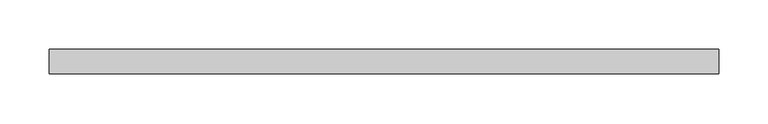
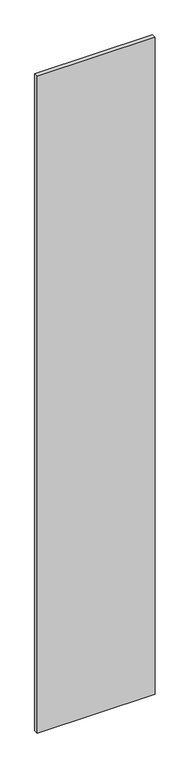
"""IFC4 building model written with IfcOpenShell, lengths in millimetres: plate geometry, 系统嵌板 : 玻璃."""

import ifcopenshell
import ifcopenshell.guid

model = None  # the IFC model being written
_history = None  # IfcOwnerHistory: only IFC2X3 demands one
_inside = {}  # id of a spatial element -> (the spatial element, [elements in it])
_under = {}  # id of a project, library or spatial element -> (it, [spatial elements below it])
_declared = {}  # id of a project -> (the project, [libraries it declares])
_typed = {}  # id of a type object -> (the type object, [elements of that type])
_made_of = {}  # id of a material, layer set ... -> (it, [elements and type objects made of it])


def new_model(schema):
    """Start an empty IFC model of exactly this schema.

    Asked for "IFC4X3", IfcOpenShell would pick the latest addendum, in which some entities
    have other attributes; the version numbers below select the first issue.
    IFC2X3 requires an IfcOwnerHistory on every rooted entity: one is made here for all.
    """
    global model, _history
    if schema == "IFC4X3":
        model = ifcopenshell.file(schema_version=(4, 3, 0, 0))
    else:
        model = ifcopenshell.file(schema=schema)
    _inside.clear()
    _under.clear()
    _declared.clear()
    _typed.clear()
    _made_of.clear()
    _history = None
    if model.schema == "IFC2X3":
        org = make("IfcOrganization", Name="unknown")
        user = make(
            "IfcPersonAndOrganization",
            ThePerson=make("IfcPerson", FamilyName="unknown"),
            TheOrganization=org,
        )
        app = make(
            "IfcApplication",
            ApplicationDeveloper=org,
            Version="unknown",
            ApplicationFullName="unknown",
            ApplicationIdentifier="unknown",
        )
        _history = make(
            "IfcOwnerHistory",
            OwningUser=user,
            OwningApplication=app,
            ChangeAction="ADDED",
            CreationDate=0,
        )
    return model


def make(cls, **values):
    """One entity of the class cls with the attributes given. An attribute that is None is left unset."""
    return model.create_entity(
        cls, **{name: value for name, value in values.items() if value is not None}
    )


def rooted(cls, **values):
    """An entity with a GlobalId (a new one), such as an element, a storey or a relation."""
    return make(cls, GlobalId=ifcopenshell.guid.new(), OwnerHistory=_history, **values)


def si_unit(unit_type, name, prefix=None):
    """IfcSIUnit, for example si_unit("LENGTHUNIT", "METRE", prefix="MILLI")."""
    return make("IfcSIUnit", UnitType=unit_type, Prefix=prefix, Name=name)


def assignment(units):
    """IfcUnitAssignment: the units of a project."""
    return None if units is None else make("IfcUnitAssignment", Units=units)


def point(xyz):
    """IfcCartesianPoint."""
    return None if xyz is None else make("IfcCartesianPoint", Coordinates=xyz)


def direction(xyz):
    """IfcDirection."""
    return None if xyz is None else make("IfcDirection", DirectionRatios=xyz)


def frame(location, z_axis=None, x_axis=None):
    """IfcAxis2Placement3D, a coordinate frame: its origin and axes. An axis left out is left unset."""
    return make(
        "IfcAxis2Placement3D",
        Location=point(location),
        Axis=direction(z_axis),
        RefDirection=direction(x_axis),
    )


def origin():
    """The frame at (0, 0, 0) with its axes left unset."""
    return frame((0.0, 0.0, 0.0))


def origin_with_axes():
    """The frame at (0, 0, 0) with the z axis (0, 0, 1) and the x axis (1, 0, 0) written out."""
    return frame((0.0, 0.0, 0.0), z_axis=(0.0, 0.0, 1.0), x_axis=(1.0, 0.0, 0.0))


def place(relative_to, where):
    """IfcLocalPlacement: puts the frame where relative to a parent placement (None: the world)."""
    return make(
        "IfcLocalPlacement", PlacementRelTo=relative_to, RelativePlacement=where
    )


def context(
    kind, dimensions, precision=None, world=None, true_north=None, identifier=None
):
    """IfcGeometricRepresentationContext, for example the 3D "Model" context."""
    return make(
        "IfcGeometricRepresentationContext",
        ContextIdentifier=identifier,
        ContextType=kind,
        CoordinateSpaceDimension=dimensions,
        Precision=precision,
        WorldCoordinateSystem=world,
        TrueNorth=true_north,
    )


def project(units=None, contexts=None):
    """IfcProject with its units and contexts."""
    return rooted(
        "IfcProject",
        Name="project",
        RepresentationContexts=contexts,
        UnitsInContext=assignment(units),
    )


def spatial(cls, under=None, at=None, **own):
    """A site, building, storey or space (cls), placed at a placement, below another one or the project."""
    s = rooted(cls, ObjectPlacement=at, **own)
    if under is not None:
        _under.setdefault(under.id(), (under, []))[1].append(s)
    return s


def polyline(points):
    """IfcPolyline through the points."""
    return make("IfcPolyline", Points=[point(p) for p in points])


def outline(outer, holes=None, kind="AREA"):
    """IfcArbitraryClosedProfileDef: a profile drawn as a closed curve; with holes, ...WithVoids."""
    if holes is None:
        return make("IfcArbitraryClosedProfileDef", ProfileType=kind, OuterCurve=outer)
    return make(
        "IfcArbitraryProfileDefWithVoids",
        ProfileType=kind,
        OuterCurve=outer,
        InnerCurves=holes,
    )


def extrude(swept, where, along, depth):
    """IfcExtrudedAreaSolid: the profile swept, set in the frame where, extruded along a direction by depth."""
    return make(
        "IfcExtrudedAreaSolid",
        SweptArea=swept,
        Position=where,
        ExtrudedDirection=direction(along),
        Depth=depth,
    )


def shape(context_of_items, identifier, shape_type, items):
    """IfcShapeRepresentation: the items that make up one representation, for example the "Body"."""
    return make(
        "IfcShapeRepresentation",
        ContextOfItems=context_of_items,
        RepresentationIdentifier=identifier,
        RepresentationType=shape_type,
        Items=items,
    )


def source(mapping_origin, context_of_items, identifier, shape_type, items):
    """IfcRepresentationMap: a shape defined once, which mapped items show again and again."""
    return make(
        "IfcRepresentationMap",
        MappingOrigin=mapping_origin,
        MappedRepresentation=shape(context_of_items, identifier, shape_type, items),
    )


def transform(
    local_origin,
    x_axis=None,
    y_axis=None,
    z_axis=None,
    scale=None,
    scale2=None,
    scale3=None,
    uniform=True,
):
    """IfcCartesianTransformationOperator3D, or its non-uniform kind. x_axis, y_axis, z_axis: its Axis1, 2, 3."""
    if uniform:
        return make(
            "IfcCartesianTransformationOperator3D",
            Axis1=direction(x_axis),
            Axis2=direction(y_axis),
            LocalOrigin=point(local_origin),
            Scale=scale,
            Axis3=direction(z_axis),
        )
    return make(
        "IfcCartesianTransformationOperator3DnonUniform",
        Axis1=direction(x_axis),
        Axis2=direction(y_axis),
        LocalOrigin=point(local_origin),
        Scale=scale,
        Axis3=direction(z_axis),
        Scale2=scale2,
        Scale3=scale3,
    )


def mapped(mapping_source, mapping_target):
    """IfcMappedItem: shows the shape of a source again, moved by a transform."""
    return make(
        "IfcMappedItem", MappingSource=mapping_source, MappingTarget=mapping_target
    )


def made_of(thing, what):
    """Note that an element or type object is made of a material, layer set ...; save() writes the relation."""
    if what is not None:
        _made_of.setdefault(what.id(), (what, []))[1].append(thing)
    return thing


def element(
    cls,
    number,
    at=None,
    inside=None,
    cuts=None,
    type_object=None,
    material=None,
    context=None,
    identifier="Body",
    shape_type=None,
    held_by="IfcProductDefinitionShape",
    body=None,
    shapes=None,
    **own,
):
    """One element of the class cls, such as IfcWall. Its Tag is "e" and its number.

    at: its placement. inside: the storey or other place that contains it. cuts: it is an
    opening in that element (IfcRelVoidsElement). A single representation is given by context,
    identifier, shape_type and body (its items); several are given by shapes. held_by: the class
    of the entity that holds the representations. save() writes the other relations.
    """
    e = rooted(cls, Tag="e%d" % number, ObjectPlacement=at, **own)
    if body is not None:
        shapes = [shape(context, identifier, shape_type, body)]
    if shapes is not None:
        e.Representation = make(held_by, Representations=shapes)
    if inside is not None:
        _inside.setdefault(inside.id(), (inside, []))[1].append(e)
    if cuts is not None:
        rooted(
            "IfcRelVoidsElement", RelatingBuildingElement=cuts, RelatedOpeningElement=e
        )
    if type_object is not None:
        _typed.setdefault(type_object.id(), (type_object, []))[1].append(e)
    return made_of(e, material)


def aggregate(whole, parts):
    """IfcRelAggregates: a whole, such as a stair, and the parts it consists of."""
    return rooted("IfcRelAggregates", RelatingObject=whole, RelatedObjects=parts)


def save(model, path):
    """Write the relations noted so far, then the file.

    IfcRelAggregates (storeys below a building ...), IfcRelContainedInSpatialStructure (elements
    in a storey), IfcRelDefinesByType, IfcRelAssociatesMaterial and IfcRelDeclares: one each for
    every whole, place, type object, material and project.
    """
    for whole, parts in _under.values():
        aggregate(whole, parts)
    for where, things in _inside.values():
        rooted(
            "IfcRelContainedInSpatialStructure",
            RelatedElements=things,
            RelatingStructure=where,
        )
    for kind, things in _typed.values():
        rooted("IfcRelDefinesByType", RelatedObjects=things, RelatingType=kind)
    for what, things in _made_of.values():
        rooted("IfcRelAssociatesMaterial", RelatedObjects=things, RelatingMaterial=what)
    for by, libraries in _declared.values():
        rooted("IfcRelDeclares", RelatingContext=by, RelatedDefinitions=libraries)
    model.write(path)


def plate_147ead81(model_context):
    return source(origin(), model_context, "Body", "SweptSolid", [
        extrude(outline(polyline([(340.0, -12.5), (-340.0, -12.5), (-340.0, 12.5), (340.0, 12.5), (340.0, -12.5)])), origin_with_axes(), (0.0, 0.0, 1.0), 4000.0),
    ])


if __name__ == "__main__":
    model = new_model("IFC4")
    model_context = context("Model", 3, world=origin())
    ifc_project = project(units=[si_unit("LENGTHUNIT", "METRE", prefix="MILLI")], contexts=[model_context])
    site = spatial("IfcSite", under=ifc_project)
    building = spatial("IfcBuilding", under=site)
    placement = place(None, origin())
    plate_shape = plate_147ead81(model_context)
    element("IfcPlate", 1, ObjectType="系统嵌板 : 玻璃", at=placement, inside=building, context=model_context, shape_type="MappedRepresentation", body=[
        mapped(plate_shape, transform((0.0, 0.0, 0.0), x_axis=(1.0, 0.0, 0.0), y_axis=(0.0, 1.0, 0.0), z_axis=(0.0, 0.0, 1.0))),
    ])
    save(model, "model.ifc")

# Revit data of these elements
# Type "系统嵌板 : 玻璃"
#   Construction Type Id = "GSP4R"
#   Analytic Construction = "1/8 英寸 Pilkington 单层玻璃"
#   Visual Light Transmittance = 0.9
#   Solar Heat Gain Coefficient = 0.86
#   Heat Transfer Coefficient (U) = 6.7069 W/(m²·K)
# Element 1 (IfcPlate, "系统嵌板 : 玻璃")
#   Materials on its faces: "玻璃"
# Materials
#   "玻璃": class "玻璃", colour RGB 0 128 192, transparency 0.9, Description = "钠钙玻璃", Cost = 0
